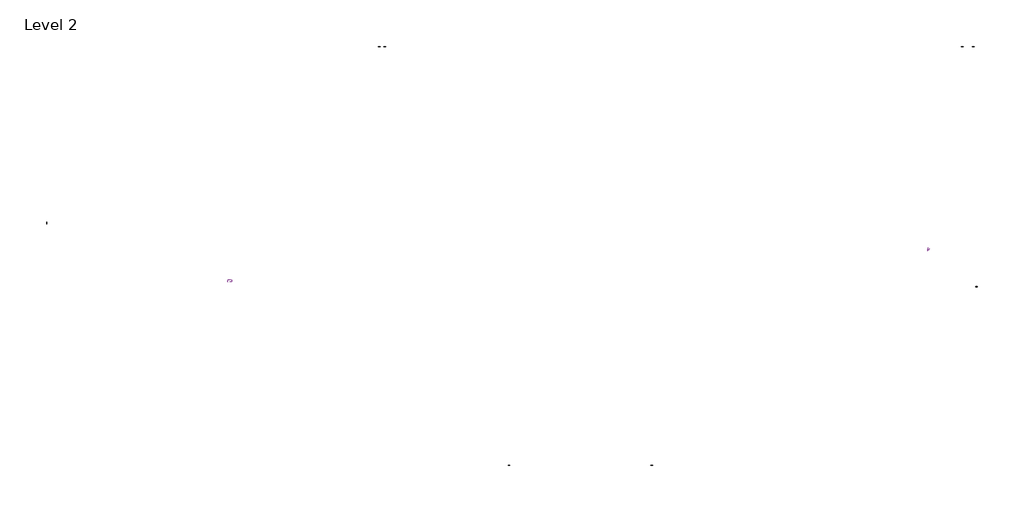
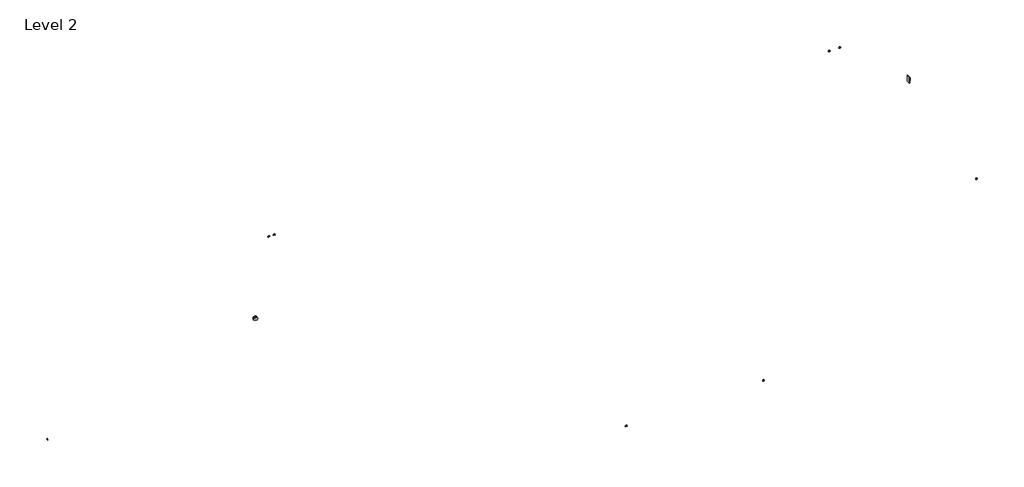
# One storey: 10 proxies.
# Revit data of these elements (continued)
# Space at (17965.722, 3358.948) mm, phase "New Construction", upper level "Level 3 Roof LP", upper offset 0 mm, lower offset 0 mm (continued)
#   Latent Heat Gain per person = 0
#   Total Heat Gain per person = 0
#   Area per Person = 0
#   Number of People = 4.57466 (stored number, unit not read)
#   COBie.Space.UsableHeight = 3500 mm
#   COBie.Space.GrossArea = 129.461 m²
#   COBie.Space.NetArea = 0 m²
#   Lighting Load Units = 0
#   Power Load Units = 0
#   Return Airflow = 0
#   Occupancy Unit = -1
#   Condition Type = 2
#   COBie = yes
#   Construction Type = none
# Space at (2061.793, 12853.016) mm, phase "New Construction", upper level "Level 3 Roof LP", upper offset 0 mm, lower offset 0 mm
#   Number = "202"
#   Name = "Storage Room"
#   Classification.Space.Number = "13-63 13 11"
#   Classification.Space.Description = "Storage Room"
#   COBie.CreatedBy = "info@mma.ie"
#   COBie.CreatedOn = "2017-07-26T09:12:43"
#   COBie.Space.Name = "202"
#   COBie.Space.Category = "13-63 13 11 : Storage Room"
#   COBie.Space.Description = "Storage Room"
#   Actual Lighting Load per area = 0
#   Actual Power Load per area = 0
#   Sensible Heat Gain per person = 0
#   Specified Lighting Load = 0
#   Specified Power Load = 0
#   Latent Heat Gain per person = 0
#   Total Heat Gain per person = 0
#   Area per Person = 0
#   Number of People = 0.601408 (stored number, unit not read)
#   COBie.Space.UsableHeight = 3500 mm
#   COBie.Space.GrossArea = 17.1831 m²
#   COBie.Space.NetArea = 0 m²
#   Lighting Load Units = 0
#   Power Load Units = 0
#   Return Airflow = 0
#   Occupancy Unit = -1
#   Condition Type = 2
#   COBie = yes
#   Construction Type = none
# Space at (6037.549, 11622.683) mm, phase "New Construction", upper level "Level 3 Roof LP", upper offset 0 mm, lower offset 0 mm
#   Number = "203"
#   Name = "Bedroom"
#   Classification.Space.Number = "13-65 19"
#   Classification.Space.Description = "Bedroom"
#   COBie.CreatedBy = "info@mma.ie"
#   COBie.CreatedOn = "2017-07-26T09:12:43"
#   COBie.Space.Name = "203"
#   COBie.Space.Category = "13-65 19 : Bedroom"
#   COBie.Space.Description = "Bedroom"
#   Actual Lighting Load per area = 0
#   Actual Power Load per area = 0
#   Sensible Heat Gain per person = 0
#   Specified Lighting Load = 0
#   Specified Power Load = 0
#   Latent Heat Gain per person = 0
#   Total Heat Gain per person = 0
#   Area per Person = 0
#   Number of People = 0.748431 (stored number, unit not read)
#   COBie.Space.UsableHeight = 3500 mm
#   COBie.Space.GrossArea = 21.3837 m²
#   COBie.Space.NetArea = 0 m²
#   Lighting Load Units = 0
#   Power Load Units = 0
#   Return Airflow = 0
#   Occupancy Unit = -1
#   Condition Type = 2
#   COBie = yes
#   Construction Type = none
# Space at (7064.002, 9552.118) mm, phase "New Construction", upper level "Level 3 Roof LP", upper offset 0 mm, lower offset 0 mm
#   Number = "204"
#   Name = "Bath"
#   Classification.Space.Number = "13-65 13"
#   Classification.Space.Description = "Bathroom"
#   COBie.CreatedBy = "info@mma.ie"
#   COBie.CreatedOn = "2017-07-26T09:12:43"
#   COBie.Space.Name = "204"
#   COBie.Space.Category = "13-65 13 : Bathroom"
#   COBie.Space.Description = "Bath"
#   Actual Lighting Load per area = 0
#   Actual Power Load per area = 0
#   Sensible Heat Gain per person = 0
#   Specified Lighting Load = 0
#   Specified Power Load = 0
#   Latent Heat Gain per person = 0
#   Total Heat Gain per person = 0
#   Area per Person = 0
#   Number of People = 0.15084 (stored number, unit not read)
#   COBie.Space.UsableHeight = 3500 mm
#   COBie.Space.GrossArea = 4.30971 m²
#   COBie.Space.NetArea = 0 m²
#   Lighting Load Units = 0
#   Power Load Units = 0
#   Return Airflow = 0
#   Occupancy Unit = -1
#   Condition Type = 2
#   COBie = yes
#   Construction Type = none
# Space at (8984.129, 9552.118) mm, phase "New Construction", upper level "Level 3 Roof LP", upper offset 0 mm, lower offset 0 mm
#   Number = "206"
#   Name = "Bath"
#   Classification.Space.Number = "13-65 13"
#   Classification.Space.Description = "Bathroom"
#   COBie.CreatedBy = "info@mma.ie"
#   COBie.CreatedOn = "2017-07-26T09:12:43"
#   COBie.Space.Name = "206"
#   COBie.Space.Category = "13-65 13 : Bathroom"
#   COBie.Space.Description = "Bath"
#   Actual Lighting Load per area = 0
#   Actual Power Load per area = 0
#   Sensible Heat Gain per person = 0
#   Specified Lighting Load = 0
#   Specified Power Load = 0
#   Latent Heat Gain per person = 0
#   Total Heat Gain per person = 0
#   Area per Person = 0
#   Number of People = 0.149872 (stored number, unit not read)
#   COBie.Space.UsableHeight = 3500 mm
#   COBie.Space.GrossArea = 4.28206 m²
#   COBie.Space.NetArea = 0 m²
#   Lighting Load Units = 0
#   Power Load Units = 0
#   Return Airflow = 0
#   Occupancy Unit = -1
#   Condition Type = 2
#   COBie = yes
#   Construction Type = none
# Space at (11964.9, 7347.683) mm, phase "New Construction", upper level "Level 3 Roof LP", upper offset 0 mm, lower offset 0 mm
#   Number = "217"
#   Name = "Hall"
#   Classification.Space.Number = "13-25 11"
#   Classification.Space.Description = "Primary Circulation Spaces"
#   COBie.CreatedBy = "info@mma.ie"
#   COBie.CreatedOn = "2017-07-26T09:12:43"
#   COBie.Space.Name = "217"
#   COBie.Space.Category = "13-25 11 : Primary Circulation Spaces"
#   COBie.Space.Description = "Hall"
#   Actual Lighting Load per area = 0
#   Actual Power Load per area = 0
#   Sensible Heat Gain per person = 0
#   Specified Lighting Load = 0
#   Specified Power Load = 0
#   Latent Heat Gain per person = 0
#   Total Heat Gain per person = 0
#   Area per Person = 0
#   Number of People = 1.45296 (stored number, unit not read)
#   COBie.Space.UsableHeight = 3500 mm
#   COBie.Space.GrossArea = 41.5133 m²
#   COBie.Space.NetArea = 0 m²
#   Lighting Load Units = 0
#   Power Load Units = 0
#   Return Airflow = 0
#   Occupancy Unit = -1
#   Condition Type = 2
#   COBie = yes
#   Construction Type = none
